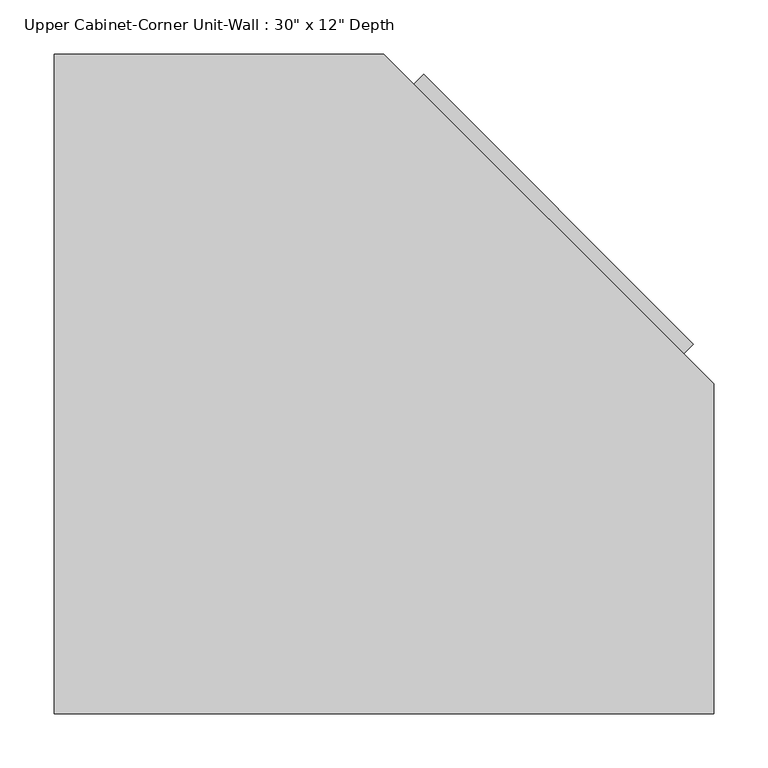
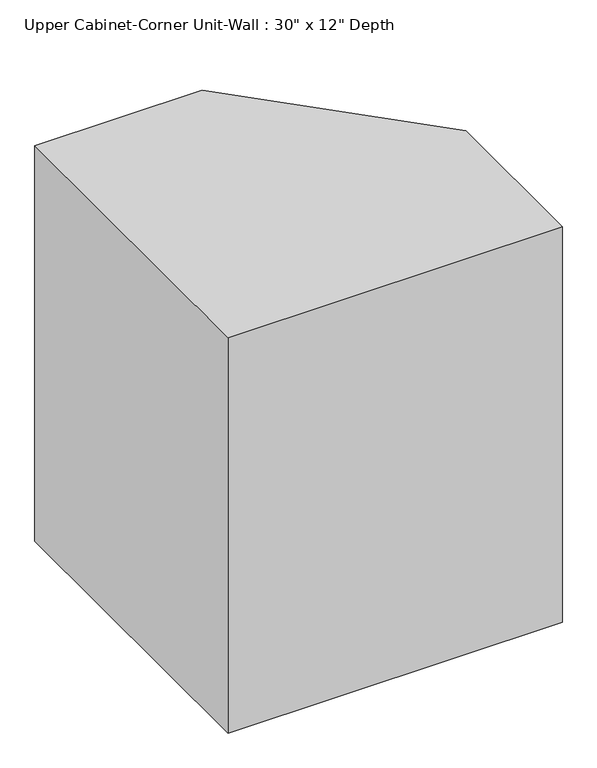
"""IFC4 building model written with IfcOpenShell, lengths in millimetres: furniture geometry."""

from ifc_helpers import new_model, si_unit, frame, origin, place, context, project, spatial, polyline, outline, extrude, faceted_brep, source, transform, mapped, element, save


def furniture_a36e1e99(model_context):
    return source(origin(), model_context, "Body", "SolidModel", [
        extrude(outline(polyline([(295.0625715, 652.7816036), (544.4402664, 403.4039087), (526.4797541, 385.4433964), (277.1020592, 634.8210913), (295.0625715, 652.7816036)])), frame((0.0, 0.0, 1733.55), z_axis=(0.0, 0.0, 1.0), x_axis=(1.0, 0.0, 0.0)), (0.0, 0.0, 1.0), 647.7),
        extrude(outline(polyline([(-27.3788372, 652.4625), (250.4803944, 652.4625), (544.1211628, 358.8217316), (544.1211628, 80.9625), (-27.3788372, 80.9625), (-27.3788372, 652.4625)])), frame((0.0, 0.0, 1676.4), z_axis=(0.0, 0.0, 1.0), x_axis=(1.0, 0.0, 0.0)), (0.0, 0.0, 1.0), 25.4),
        faceted_brep([(-46.4288372, 671.5125, 1676.4), (258.3711628, 671.5125, 1676.4), (563.1711628, 366.7125, 1676.4), (563.1711628, 61.9125, 1676.4), (-46.4288372, 61.9125, 1676.4), (250.4803944, 652.4625, 1676.4), (-27.3788372, 652.4625, 1676.4), (-27.3788372, 80.9625, 1676.4), (544.1211628, 80.9625, 1676.4), (544.1211628, 358.8217316, 1676.4), (-46.4288372, 671.5125, 2438.4), (-46.4288372, 61.9125, 2438.4), (563.1711628, 61.9125, 2438.4), (563.1711628, 366.7125, 2438.4), (258.3711628, 671.5125, 2438.4), (250.4803944, 652.4625, 2413.0), (-27.3788372, 652.4625, 2413.0), (-27.3788372, 80.9625, 2413.0), (544.1211628, 80.9625, 2413.0), (544.1211628, 358.8217316, 2413.0), (535.4600102, 394.4236525, 2381.25), (286.0823153, 643.8013475, 2381.25), (286.0823153, 643.8013475, 1733.55), (535.4600102, 394.4236525, 1733.55), (272.6119312, 630.3309633, 2381.25), (521.9896261, 380.9532684, 2381.25), (521.9896261, 380.9532684, 1733.55), (272.6119312, 630.3309633, 1733.55)], [[[0, 1, 2, 3, 4], [5, 6, 7, 8, 9]], [[10, 11, 12, 13, 14]], [[1, 0, 10, 14]], [[6, 5, 15, 16]], [[7, 6, 16, 17]], [[8, 7, 17, 18]], [[9, 8, 18, 19]], [[3, 2, 13, 12]], [[4, 3, 12, 11]], [[0, 4, 11, 10]], [[16, 15, 19, 18, 17]], [[2, 1, 14, 13], [20, 21, 22, 23]], [[5, 9, 19, 15], [24, 25, 26, 27]], [[20, 25, 24, 21]], [[22, 27, 26, 23]], [[21, 24, 27, 22]], [[25, 20, 23, 26]]]),
    ])


if __name__ == "__main__":
    model = new_model("IFC4")
    model_context = context("Model", 3, world=origin())
    ifc_project = project(units=[si_unit("LENGTHUNIT", "METRE", prefix="MILLI")], contexts=[model_context])
    site = spatial("IfcSite", under=ifc_project)
    building = spatial("IfcBuilding", under=site)
    placement = place(None, origin())
    furniture_shape = furniture_a36e1e99(model_context)
    element("IfcFurniture", 1, ObjectType="Upper Cabinet-Corner Unit-Wall : 30\" x 12\" Depth", at=placement, inside=building, context=model_context, shape_type="MappedRepresentation", body=[
        mapped(furniture_shape, transform((0.0, 0.0, 0.0), x_axis=(1.0, 0.0, 0.0), y_axis=(0.0, 1.0, 0.0), z_axis=(0.0, 0.0, 1.0))),
    ])
    save(model, "model.ifc")

# Revit data of these elements
# Type "Upper Cabinet-Corner Unit-Wall : 30\" x 12\" Depth"
#   Assembly Code = "C1030410"
#   Depth = 1' - 0"
#   Height = 2' - 6"
#   Top of Cabinet = 8' - 0"
#   Width = 0' - 2"
#   COBie.Type = no
#   Cabinet Material = none
#   Door/Drawer Material = none
# Element 1 (IfcFurniture, "Upper Cabinet-Corner Unit-Wall : 30\" x 12\" Depth")
#   Materials on its faces: "Cabinets"
# Materials
#   "Cabinets": class "Miscellaneous", colour RGB 249 249 249, transparency 0
